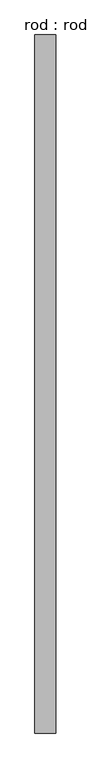
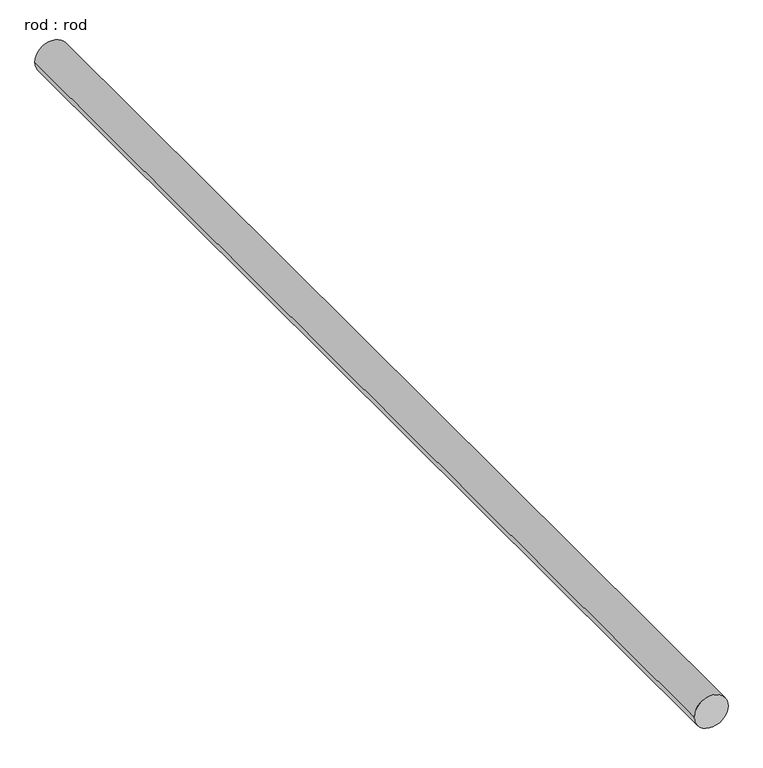
"""IFC4 building model written with IfcOpenShell, lengths in millimetres: proxy geometry, rod : rod."""

from ifc_helpers import new_model, si_unit, point, frame, frame_2d, origin, place, context, project, spatial, circle_curve, trimmed, segment, composite_curve, outline, extrude, source, transform, mapped, element, save


def rod_rod_5b457a64(model_context):
    return source(origin(), model_context, "Body", "SweptSolid", [
        extrude(outline(composite_curve([segment(trimmed(circle_curve(frame_2d((0.0108462, 0.0)), 200.0), [point((0.0108462, 200.0))], [point((0.0108462, -200.0))], False, "CARTESIAN"), True, "CONTINUOUS"), segment(trimmed(circle_curve(frame_2d((0.0108462, 0.0)), 200.0), [point((0.0108462, -200.0))], [point((0.0108462, 200.0))], False, "CARTESIAN"), True, "CONTINUOUS")], self_intersect=False)), frame((0.0, -2657.7547007, 0.0), z_axis=(0.0, 1.0, 0.0), x_axis=(0.0, 0.0, 1.0)), (0.0, 0.0, 1.0), 13500.9666321),
    ])


if __name__ == "__main__":
    model = new_model("IFC4")
    model_context = context("Model", 3, world=origin())
    ifc_project = project(units=[si_unit("LENGTHUNIT", "METRE", prefix="MILLI")], contexts=[model_context])
    site = spatial("IfcSite", under=ifc_project)
    building = spatial("IfcBuilding", under=site)
    placement = place(None, origin())
    rod_rod_shape = rod_rod_5b457a64(model_context)
    element("IfcBuildingElementProxy", 1, Name="rod : rod", ObjectType="rod : rod", at=placement, inside=building, context=model_context, shape_type="MappedRepresentation", body=[
        mapped(rod_rod_shape, transform((0.0, 0.0, 0.0), x_axis=(1.0, 0.0, 0.0), y_axis=(0.0, 1.0, 0.0), z_axis=(0.0, 0.0, 1.0))),
    ])
    save(model, "model.ifc")

# Revit data of these elements
# Type "rod : rod"
#   Default Elevation = 0
